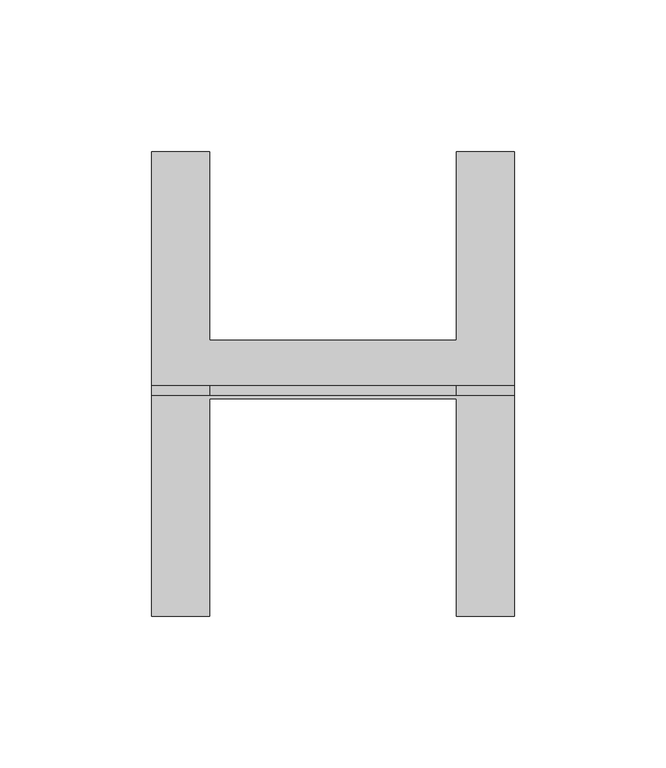
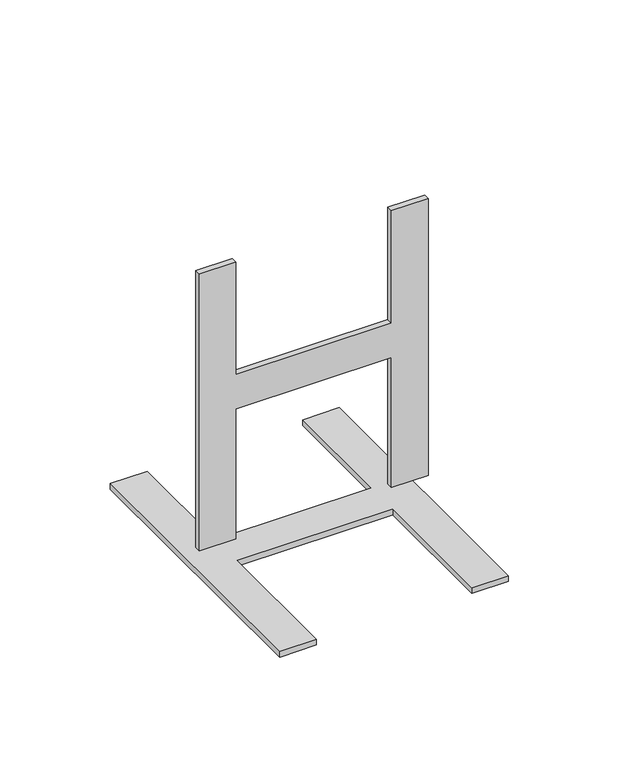
"""IFC4 building model written with IfcOpenShell, lengths in millimetres: proxy geometry, Grid Number1_FedEx : Grid Number1_FedEx."""

from ifc_helpers import new_model, si_unit, frame, origin, origin_with_axes, place, context, project, spatial, polyline, outline, extrude, source, transform, mapped, element, save


def entourage_c0d9e6b8(model_context):
    return source(origin(), model_context, "Body", "SweptSolid", [
        extrude(outline(polyline([(-167.8768239, 146.5840649), (-167.8768239, 299.6794816), (-148.7398968, 299.6794816), (-148.7398968, 237.4844686), (-67.4079567, 237.4844686), (-67.4079567, 299.6794816), (-48.2710296, 299.6794816), (-48.2710296, 146.5840649), (-67.4079567, 146.5840649), (-67.4079567, 218.3475415), (-148.7398968, 218.3475415), (-148.7398968, 146.5840649), (-167.8768239, 146.5840649)])), origin_with_axes(), (0.0, 0.0, 1.0), 3.175),
        extrude(outline(polyline([(14.4798932, -167.8768239), (14.4798932, -148.7398968), (86.2433698, -148.7398968), (86.2433698, -67.4079567), (14.4798932, -67.4079567), (14.4798932, -48.2710296), (167.5753099, -48.2710296), (167.5753099, -67.4079567), (105.3802969, -67.4079567), (105.3802969, -148.7398968), (167.5753099, -148.7398968), (167.5753099, -167.8768239), (14.4798932, -167.8768239)])), frame((0.0, 219.3456765, 0.0), z_axis=(0.0, 1.0, 0.0), x_axis=(0.0, 0.0, 1.0)), (0.0, 0.0, 1.0), 3.175),
    ])


if __name__ == "__main__":
    model = new_model("IFC4")
    model_context = context("Model", 3, world=origin())
    ifc_project = project(units=[si_unit("LENGTHUNIT", "METRE", prefix="MILLI")], contexts=[model_context])
    site = spatial("IfcSite", under=ifc_project)
    building = spatial("IfcBuilding", under=site)
    placement = place(None, origin())
    entourage_shape = entourage_c0d9e6b8(model_context)
    element("IfcBuildingElementProxy", 1, Name="Grid Number1_FedEx : Grid Number1_FedEx", ObjectType="Grid Number1_FedEx : Grid Number1_FedEx", at=placement, inside=building, context=model_context, shape_type="MappedRepresentation", body=[
        mapped(entourage_shape, transform((0.0, 0.0, 0.0), x_axis=(1.0, 0.0, 0.0), y_axis=(0.0, 1.0, 0.0), z_axis=(0.0, 0.0, 1.0))),
    ])
    save(model, "model.ifc")

# Revit data of these elements
# Type "Grid Number1_FedEx : Grid Number1_FedEx"
#   Grid [instance default] = "S.8"
#   Label Width [instance default] = 1' - 0"
#   Half Box Width2 [instance default] = 0' - 6.13846"
#   Half Box Width [instance default] = 0' - 6"
#   Robust [instance default] = yes
#   Height = 0
#   Assembly Code = ""
# Element 1 (IfcBuildingElementProxy, "Grid Number1_FedEx : Grid Number1_FedEx")
#   Grid = "H"
#   Robust = no
#   Materials on its faces: "Letter"
# Materials
#   "Letter": class "Unassigned", colour RGB 178 187 30, transparency 0, Comments = "Rendering appearance not upgraded "
